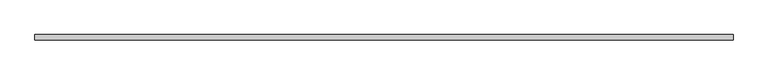
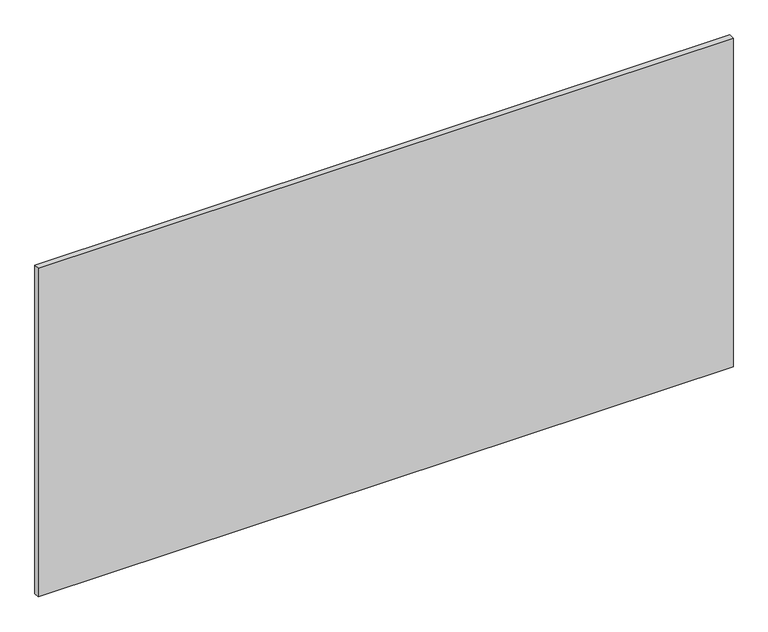
"""IFC4 building model written with IfcOpenShell, lengths in millimetres: proxy geometry, Inner panel:Inner panel:1:Inner panel:1 : Inner panel:Inner panel:300324:300043:Inner panel:1:Inner panel:1 : Inner panel:Inner panel:300324:300043 : Inner panel:Inner panel:1:Inner panel:1 : Inner panel:Inner panel:300324:300043:38 : Inner panel:Inner panel:1:Inner panel:1 : Inner panel:Inner panel:300324:300043:Inner panel:1:Inner panel:1 : Inner panel:Inner panel:300324:300043 : Inner panel:Inner panel:1:Inner panel:1 : Inner panel:Inner panel:300324:300043:300031."""

from ifc_helpers import new_model, si_unit, frame, origin, place, context, project, spatial, polyline, outline, extrude, source, transform, mapped, element, save


def generic_models_668c35f7(model_context):
    return source(origin(), model_context, "Body", "SweptSolid", [
        extrude(outline(polyline([(568007.8867239, -578778.4413841), (570446.2867239, -578778.4413841), (570446.2867239, -578797.4913841), (568007.8867239, -578797.4913841), (568007.8867239, -578778.4413841)])), frame((0.0, 0.0, 3721.1), z_axis=(0.0, 0.0, 1.0), x_axis=(1.0, 0.0, 0.0)), (0.0, 0.0, 1.0), 1219.2),
    ])


if __name__ == "__main__":
    model = new_model("IFC4")
    model_context = context("Model", 3, world=origin())
    ifc_project = project(units=[si_unit("LENGTHUNIT", "METRE", prefix="MILLI")], contexts=[model_context])
    site = spatial("IfcSite", under=ifc_project)
    building = spatial("IfcBuilding", under=site)
    placement = place(None, origin())
    generic_models_shape = generic_models_668c35f7(model_context)
    element("IfcBuildingElementProxy", 1, Name="Inner panel:Inner panel:1:Inner panel:1 : Inner panel:Inner panel:300324:300043:Inner panel:1:Inner panel:1 : Inner panel:Inner panel:300324:300043 : Inner panel:Inner panel:1:Inner panel:1 : Inner panel:Inner panel:300324:300043:38 : Inner panel:Inner panel:1:Inner panel:1 : Inner panel:Inner panel:300324:300043:Inner panel:1:Inner panel:1 : Inner panel:Inner panel:300324:300043 : Inner panel:Inner panel:1:Inner panel:1 : Inner panel:Inner panel:300324:300043:300031", ObjectType="Inner panel:Inner panel:1:Inner panel:1 : Inner panel:Inner panel:300324:300043:Inner panel:1:Inner panel:1 : Inner panel:Inner panel:300324:300043 : Inner panel:Inner panel:1:Inner panel:1 : Inner panel:Inner panel:300324:300043:38 : Inner panel:Inner panel:1:Inner panel:1 : Inner panel:Inner panel:300324:300043:Inner panel:1:Inner panel:1 : Inner panel:Inner panel:300324:300043 : Inner panel:Inner panel:1:Inner panel:1 : Inner panel:Inner panel:300324:300043:300031", at=placement, inside=building, context=model_context, shape_type="MappedRepresentation", body=[
        mapped(generic_models_shape, transform((0.0, 0.0, 0.0), x_axis=(1.0, 0.0, 0.0), y_axis=(0.0, 1.0, 0.0), z_axis=(0.0, 0.0, 1.0))),
    ])
    save(model, "model.ifc")

# Revit data of these elements
# Type "Inner panel:Inner panel:1:Inner panel:1 : Inner panel:Inner panel:300324:300043:Inner panel:1:Inner panel:1 : Inner panel:Inner panel:300324:300043 : Inner panel:Inner panel:1:Inner panel:1 : Inner panel:Inner panel:300324:300043:38 : Inner panel:Inner panel:1:Inner panel:1 : Inner panel:Inner panel:300324:300043:Inner panel:1:Inner panel:1 : Inner panel:Inner panel:300324:300043 : Inner panel:Inner panel:1:Inner panel:1 : Inner panel:Inner panel:300324:300043:300031"
#   NameOverride = "Inner panel:Inner panel:1:Inner panel:1 : Inner panel:Inner panel:300324:300043:Inner panel:1:Inner panel:1 : Inner panel:Inner panel:300324:300043 : Inner panel:Inner panel:1:Inner panel:1 : Inner panel:Inner panel:300324:300043:300031"
#   ObjectTypeOverride = "Inner panel:1:Inner panel:1 : Inner panel:Inner panel:300324:300043 : Inner panel:Inner panel:1:Inner panel:1 : Inner panel:Inner panel:300324:300043"
#   Reference = "Inner panel"
#   Tag = "300031"
# Element 1 (IfcBuildingElementProxy, "Inner panel:Inner panel:1:Inner panel:1 : Inner panel:Inner panel:300324:300043:Inner panel:1:Inner panel:1 : Inner panel:Inner panel:300324:300043 : Inner panel:Inner panel:1:Inner panel:1 : Inner panel:Inner panel:300324:300043:38 : Inner panel:Inner panel:1:Inner panel:1 : Inner panel:Inner panel:300324:300043:Inner panel:1:Inner panel:1 : Inner panel:Inner panel:300324:300043 : Inner panel:Inner panel:1:Inner panel:1 : Inner panel:Inner panel:300324:300043:300031")
#   Materials on its faces: "3/4\" PREFINISHED STAINED/SEALED PLYWOOD (FINISH: GRADE B,  FLAME SPREAD: CLASS B)"
# Materials
#   "3/4\" PREFINISHED STAINED/SEALED PLYWOOD (FINISH: GRADE B,  FLAME SPREAD: CLASS B)": class "Wood", colour RGB 149 120 74, transparency 0, Description = "Plywood, sheathing grade", Cost = 0
